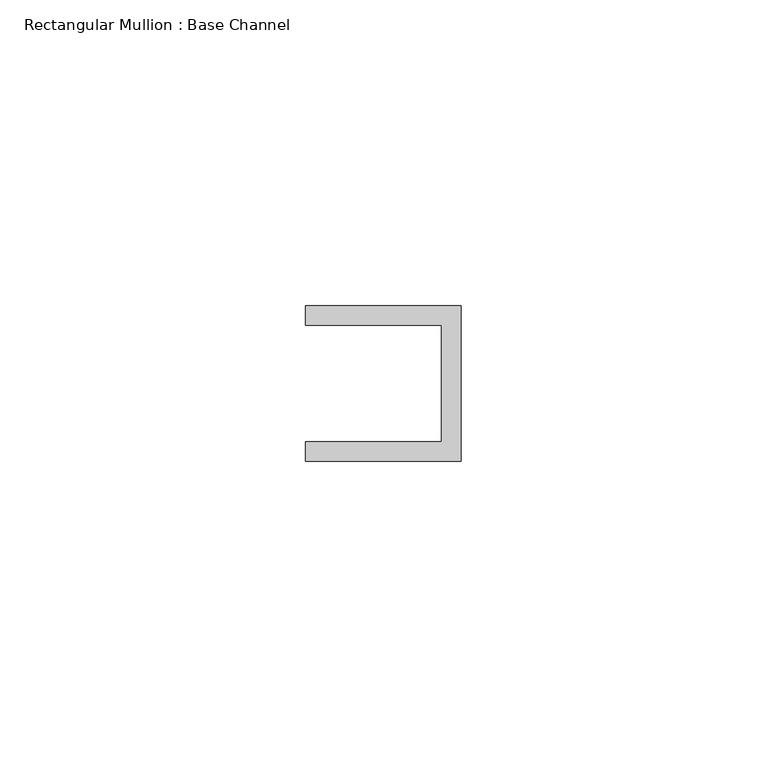
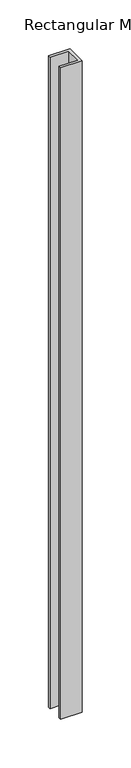
"""IFC4 building model written with IfcOpenShell, lengths in millimetres: member geometry, Rectangular Mullion : Base Channel."""

from ifc_helpers import new_model, si_unit, frame, origin, place, context, project, spatial, polyline, outline, extrude, source, transform, mapped, element, save


def rectangular_mullion_base_channel_31779efc(model_context):
    return source(origin(), model_context, "Body", "SweptSolid", [
        extrude(outline(polyline([(0.0, -12.7), (-25.4, -12.7), (-25.4, -9.525), (-3.175, -9.525), (-3.175, 9.525), (-25.4, 9.525), (-25.4, 12.7), (0.0, 12.7), (0.0, -12.7)])), frame((0.0, 0.0, -817.5625), z_axis=(0.0, 0.0, 1.0), x_axis=(1.0, 0.0, 0.0)), (0.0, 0.0, 1.0), 817.5625),
    ])


if __name__ == "__main__":
    model = new_model("IFC4")
    model_context = context("Model", 3, world=origin())
    ifc_project = project(units=[si_unit("LENGTHUNIT", "METRE", prefix="MILLI")], contexts=[model_context])
    site = spatial("IfcSite", under=ifc_project)
    building = spatial("IfcBuilding", under=site)
    placement = place(None, origin())
    rectangular_mullion_base_channel_shape = rectangular_mullion_base_channel_31779efc(model_context)
    element("IfcMember", 1, ObjectType="Rectangular Mullion : Base Channel", at=placement, inside=building, context=model_context, shape_type="MappedRepresentation", body=[
        mapped(rectangular_mullion_base_channel_shape, transform((0.0, 0.0, 0.0), x_axis=(1.0, 0.0, 0.0), y_axis=(0.0, 1.0, 0.0), z_axis=(0.0, 0.0, 1.0))),
    ])
    save(model, "model.ifc")

# Revit data of these elements
# Type "Rectangular Mullion : Base Channel"
#   built-in parameter 1007322 = 0.0833333 (stored number, unit not read)
#   built-in parameter 1007321 = 0.0416667 (stored number, unit not read)
#   built-in parameter 1007320 = -0.03125 (stored number, unit not read)
# Element 1 (IfcMember, "Rectangular Mullion : Base Channel")
#   Materials on its faces: "ALUM"
# Materials
#   "ALUM": class "Generic", colour RGB 157 157 157, transparency 0, Cost = 0
